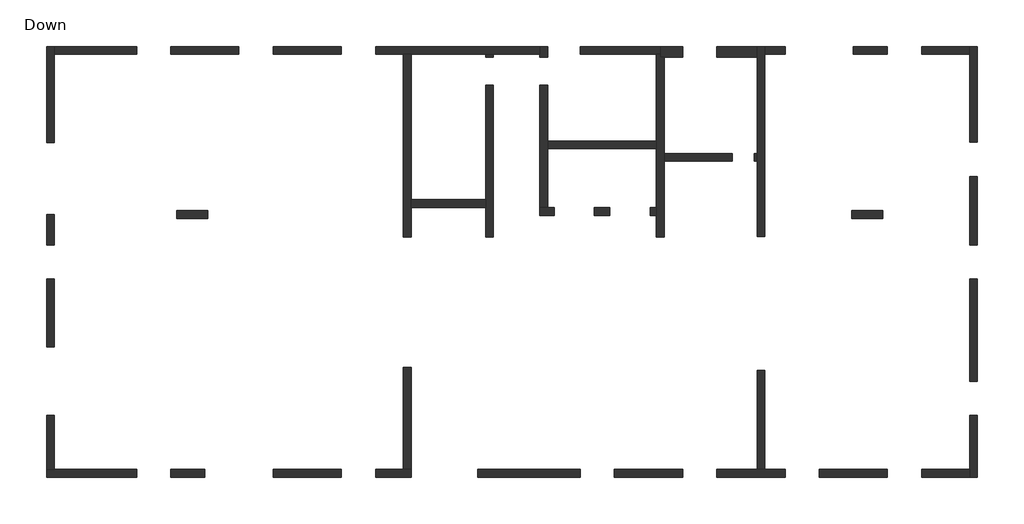
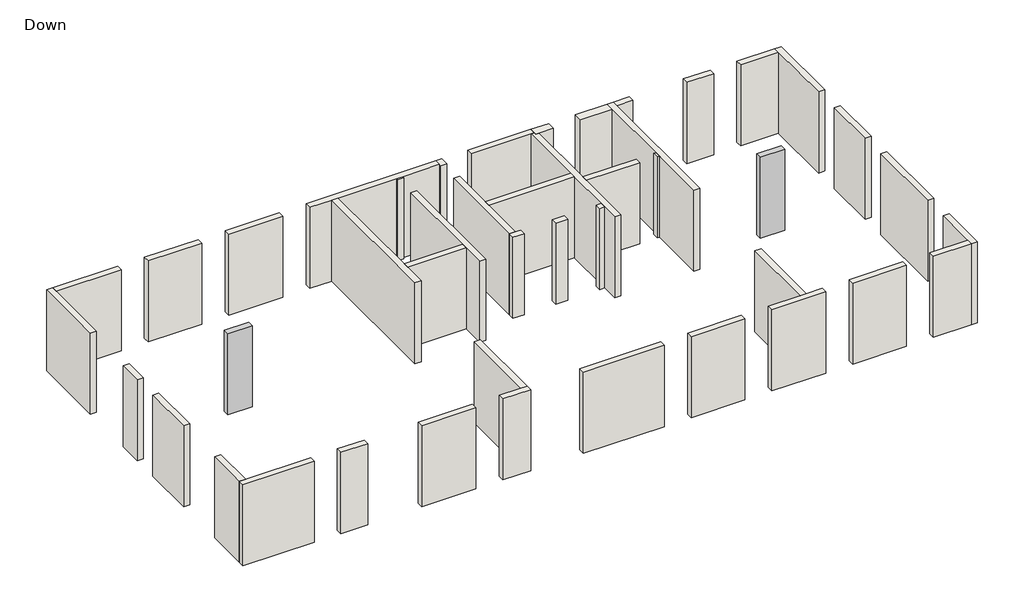
# One storey: 43 walls, 2 columns.
"""IFC4 building model written with IfcOpenShell, lengths in millimetres."""

from ifc_helpers import new_model, si_unit, origin, origin_with_axes, place, context, project, spatial, polyline, outline, extrude, faceted_brep, element, save

model = new_model("IFC4")

# Units and contexts
model_context = context("Model", 3, world=origin())
ifc_project = project(units=[si_unit("LENGTHUNIT", "METRE", prefix="MILLI")], contexts=[model_context])

# Site, building, storey
site = spatial("IfcSite", under=ifc_project)
building = spatial("IfcBuilding", under=site)
storey = spatial("IfcBuildingStorey", under=building, Name="Down", Elevation=0.0)

# Columns
placement = place(None, origin())
element("IfcColumn", 1, ObjectType="Concrete Rectengular Column : 100/25", at=placement, inside=storey, context=model_context, shape_type="Brep", body=[
    faceted_brep([(-7230.8224108, 3391.6516226, 0.0), (-6230.8224108, 3391.6516226, 0.0), (-6230.8224108, 3141.6516226, 0.0), (-7230.8224108, 3141.6516226, 0.0), (-7230.8224108, 3391.6516226, 3500.0), (-6230.8224108, 3391.6516226, 3500.0), (-6230.8224108, 3391.6516226, 3290.0), (-7230.8224108, 3391.6516226, 3290.0), (-6230.8224108, 3141.6516226, 3500.0), (-6230.8224108, 3141.6516226, 3290.0), (-7230.8224108, 3141.6516226, 3500.0), (-7230.8224108, 3141.6516226, 3290.0)], [[[0, 1, 2, 3]], [[4, 5, 6, 1, 0, 7]], [[5, 8, 9, 2, 1, 6]], [[8, 10, 11, 3, 2, 9]], [[10, 4, 7, 0, 3, 11]], [[4, 10, 8, 5]]]),
])
element("IfcColumn", 2, ObjectType="Concrete Rectengular Column : 100/25", at=placement, inside=storey, context=model_context, shape_type="Brep", body=[
    faceted_brep([(14515.7915847, 3391.6516226, 0.0), (15515.7915847, 3391.6516226, 0.0), (15515.7915847, 3141.6516226, 0.0), (14515.7915847, 3141.6516226, 0.0), (14515.7915847, 3391.6516226, 3500.0), (15515.7915847, 3391.6516226, 3500.0), (15515.7915847, 3391.6516226, 3290.0), (14515.7915847, 3391.6516226, 3290.0), (15515.7915847, 3141.6516226, 3500.0), (15515.7915847, 3141.6516226, 3290.0), (14515.7915847, 3141.6516226, 3500.0), (14515.7915847, 3141.6516226, 3290.0)], [[[0, 1, 2, 3]], [[4, 5, 6, 1, 0, 7]], [[5, 8, 9, 2, 1, 6]], [[8, 10, 11, 3, 2, 9]], [[10, 4, 7, 0, 3, 11]], [[4, 10, 8, 5]]]),
])

# Walls
element("IfcWall", 3, ObjectType="25", at=placement, inside=storey, context=model_context, shape_type="Brep", body=[
    faceted_brep([(18317.4281535, 8690.4665211, 0.0), (18317.4281535, 8440.4665211, 0.0), (18317.4281535, 5600.7374014, 0.0), (18317.4281535, 5600.7374014, 3500.0), (18317.4281535, 8440.4665211, 3500.0), (18317.4281535, 8690.4665211, 3500.0), (18567.4281535, 8690.4665211, 0.0), (18567.4281535, 8690.4665211, 3500.0), (18567.4281535, 5600.7374014, 3500.0), (18567.4281535, 5600.7374014, 0.0)], [[[0, 1, 2, 3, 4, 5]], [[6, 7, 8, 9]], [[2, 1, 0, 6, 9]], [[3, 2, 9, 8]], [[5, 4, 3, 8, 7]], [[0, 5, 7, 6]]]),
])
element("IfcWall", 4, ObjectType="25", at=placement, inside=storey, context=model_context, shape_type="SweptSolid", body=[
    extrude(outline(polyline([(18317.4281535, 2290.9179883), (18317.4281535, 4491.8209229), (18567.4281535, 4491.8209229), (18567.4281535, 2290.9179883), (18317.4281535, 2290.9179883)])), origin_with_axes(), (0.0, 0.0, 1.0), 3500.0),
])
element("IfcWall", 5, ObjectType="25", at=placement, inside=storey, context=model_context, shape_type="SweptSolid", body=[
    extrude(outline(polyline([(18317.4281535, -2106.6553751), (18317.4281535, 1194.6990267), (18567.4281535, 1194.6990267), (18567.4281535, -2106.6553751), (18317.4281535, -2106.6553751)])), origin_with_axes(), (0.0, 0.0, 1.0), 3500.0),
])
element("IfcWall", 6, ObjectType="25", at=placement, inside=storey, context=model_context, shape_type="Brep", body=[
    faceted_brep([(18317.4281535, -3207.1068424, 0.0), (18317.4281535, -4954.849506, 0.0), (18317.4281535, -5204.849506, 0.0), (18317.4281535, -5204.849506, 3500.0), (18317.4281535, -4954.849506, 3500.0), (18317.4281535, -3207.1068424, 3500.0), (18567.4281535, -3207.1068424, 0.0), (18567.4281535, -3207.1068424, 3500.0), (18567.4281535, -5204.849506, 3500.0), (18567.4281535, -5204.849506, 0.0)], [[[0, 1, 2, 3, 4, 5]], [[6, 7, 8, 9]], [[2, 1, 0, 6, 9]], [[5, 4, 3, 8, 7]], [[0, 5, 7, 6]], [[3, 2, 9, 8]]]),
])
element("IfcWall", 7, ObjectType="25", at=placement, inside=storey, context=model_context, shape_type="Brep", body=[
    faceted_brep([(18317.4281535, -4954.849506, 0.0), (16768.6132551, -4954.849506, 0.0), (16768.6132551, -4954.849506, 3500.0), (18317.4281535, -4954.849506, 3500.0), (18317.4281535, -4954.849506, 3290.0), (18317.4281535, -5204.849506, 0.0), (18317.4281535, -5204.849506, 3500.0), (16768.6132551, -5204.849506, 3500.0), (16768.6132551, -5204.849506, 0.0)], [[[0, 1, 2, 3, 4]], [[5, 6, 7, 8]], [[1, 0, 5, 8]], [[2, 1, 8, 7]], [[3, 2, 7, 6]], [[0, 4, 3, 6, 5]]]),
])
element("IfcWall", 8, ObjectType="25", at=placement, inside=storey, context=model_context, shape_type="SweptSolid", body=[
    extrude(outline(polyline([(13467.2588533, -4954.849506), (15668.1617879, -4954.849506), (15668.1617879, -5204.849506), (13467.2588533, -5204.849506), (13467.2588533, -4954.849506)])), origin_with_axes(), (0.0, 0.0, 1.0), 3500.0),
])
element("IfcWall", 9, ObjectType="25", at=placement, inside=storey, context=model_context, shape_type="Brep", body=[
    faceted_brep([(12366.8073861, -4954.849506, 0.0), (11719.2340226, -4954.849506, 0.0), (11469.2340226, -4954.849506, 0.0), (10165.9044515, -4954.849506, 0.0), (10165.9044515, -4954.849506, 3500.0), (11469.2340226, -4954.849506, 3500.0), (11719.2340226, -4954.849506, 3500.0), (12366.8073861, -4954.849506, 3500.0), (12366.8073861, -5204.849506, 0.0), (12366.8073861, -5204.849506, 3500.0), (10165.9044515, -5204.849506, 3500.0), (10165.9044515, -5204.849506, 0.0)], [[[0, 1, 2, 3, 4, 5, 6, 7]], [[8, 9, 10, 11]], [[3, 2, 1, 0, 8, 11]], [[4, 3, 11, 10]], [[7, 6, 5, 4, 10, 9]], [[0, 7, 9, 8]]]),
])
element("IfcWall", 10, ObjectType="25", at=placement, inside=storey, context=model_context, shape_type="SweptSolid", body=[
    extrude(outline(polyline([(6868.7825554, -4954.849506), (9069.6854899, -4954.849506), (9069.6854899, -5204.849506), (6868.7825554, -5204.849506), (6868.7825554, -4954.849506)])), origin_with_axes(), (0.0, 0.0, 1.0), 3500.0),
])
element("IfcWall", 11, ObjectType="25", at=placement, inside=storey, context=model_context, shape_type="SweptSolid", body=[
    extrude(outline(polyline([(2466.9766863, -4954.849506), (5768.3310881, -4954.849506), (5768.3310881, -5204.849506), (2466.9766863, -5204.849506), (2466.9766863, -4954.849506)])), origin_with_axes(), (0.0, 0.0, 1.0), 3500.0),
])
element("IfcWall", 12, ObjectType="25", at=placement, inside=storey, context=model_context, shape_type="Brep", body=[
    faceted_brep([(317.1459865, -4954.849506, 0.0), (67.1459865, -4954.849506, 0.0), (-830.1452099, -4954.849506, 0.0), (-830.1452099, -4954.849506, 3500.0), (67.1459865, -4954.849506, 3500.0), (317.1459865, -4954.849506, 3500.0), (317.1459865, -5204.849506, 0.0), (317.1459865, -5204.849506, 3500.0), (-830.1452099, -5204.849506, 3500.0), (-830.1452099, -5204.849506, 0.0)], [[[0, 1, 2, 3, 4, 5]], [[6, 7, 8, 9]], [[2, 1, 0, 6, 9]], [[3, 2, 9, 8]], [[5, 4, 3, 8, 7]], [[0, 5, 7, 6]]]),
])
element("IfcWall", 13, ObjectType="25", at=placement, inside=storey, context=model_context, shape_type="SweptSolid", body=[
    extrude(outline(polyline([(-4131.4996117, -4954.849506), (-1930.5966772, -4954.849506), (-1930.5966772, -5204.849506), (-4131.4996117, -5204.849506), (-4131.4996117, -4954.849506)])), origin_with_axes(), (0.0, 0.0, 1.0), 3500.0),
])
element("IfcWall", 14, ObjectType="25", at=placement, inside=storey, context=model_context, shape_type="SweptSolid", body=[
    extrude(outline(polyline([(-7432.8540135, -4954.849506), (-6332.4025462, -4954.849506), (-6332.4025462, -5204.849506), (-7432.8540135, -5204.849506), (-7432.8540135, -4954.849506)])), origin_with_axes(), (0.0, 0.0, 1.0), 3500.0),
])
element("IfcWall", 15, ObjectType="25", at=placement, inside=storey, context=model_context, shape_type="Brep", body=[
    faceted_brep([(-8529.0729751, -4954.849506, 0.0), (-11182.5718465, -4954.849506, 0.0), (-11432.5718465, -4954.849506, 0.0), (-11432.5718465, -4954.849506, 3500.0), (-11182.5718465, -4954.849506, 3500.0), (-8529.0729751, -4954.849506, 3500.0), (-8529.0729751, -5204.849506, 0.0), (-8529.0729751, -5204.849506, 3500.0), (-11432.5718465, -5204.849506, 3500.0), (-11432.5718465, -5204.849506, 0.0)], [[[0, 1, 2, 3, 4, 5]], [[6, 7, 8, 9]], [[2, 1, 0, 6, 9]], [[5, 4, 3, 8, 7]], [[0, 5, 7, 6]], [[3, 2, 9, 8]]]),
])
element("IfcWall", 16, ObjectType="25", at=placement, inside=storey, context=model_context, shape_type="Brep", body=[
    faceted_brep([(-11182.5718465, -4954.849506, 0.0), (-11182.5718465, -3207.1068424, 0.0), (-11182.5718465, -3207.1068424, 3290.0), (-11182.5718465, -3207.1068424, 3500.0), (-11182.5718465, -4954.849506, 3500.0), (-11182.5718465, -4954.849506, 3290.0), (-11432.5718465, -4954.849506, 0.0), (-11432.5718465, -4954.849506, 3500.0), (-11432.5718465, -3207.1068424, 3500.0), (-11432.5718465, -3207.1068424, 0.0), (-11187.5718465, -3207.1068424, 3500.0)], [[[0, 1, 2, 3, 4, 5]], [[6, 7, 8, 9]], [[1, 0, 6, 9]], [[3, 2, 1, 9, 8, 10]], [[4, 3, 10, 8, 7]], [[0, 5, 4, 7, 6]]]),
])
element("IfcWall", 17, ObjectType="25", at=placement, inside=storey, context=model_context, shape_type="Brep", body=[
    faceted_brep([(-11182.5718465, -1006.2039078, 0.0), (-11182.5718465, 1194.6990267, 0.0), (-11182.5718465, 1194.6990267, 3290.0), (-11182.5718465, 1194.6990267, 3500.0), (-11182.5718465, -1006.2039078, 3500.0), (-11182.5718465, -1006.2039078, 3290.0), (-11432.5718465, -1006.2039078, 0.0), (-11432.5718465, -1006.2039078, 3500.0), (-11432.5718465, 1194.6990267, 3500.0), (-11432.5718465, 1194.6990267, 0.0), (-11187.5718465, 1194.6990267, 3500.0), (-11187.5718465, -1006.2039078, 3500.0)], [[[0, 1, 2, 3, 4, 5]], [[6, 7, 8, 9]], [[1, 0, 6, 9]], [[3, 2, 1, 9, 8, 10]], [[4, 3, 10, 8, 7, 11]], [[0, 5, 4, 11, 7, 6]]]),
])
element("IfcWall", 18, ObjectType="25", at=placement, inside=storey, context=model_context, shape_type="Brep", body=[
    faceted_brep([(-11182.5718465, 2290.9179883, 0.0), (-11182.5718465, 3268.626792, 0.0), (-11182.5718465, 3268.626792, 3290.0), (-11182.5718465, 3268.626792, 3500.0), (-11182.5718465, 2290.9179883, 3500.0), (-11182.5718465, 2290.9179883, 3290.0), (-11432.5718465, 2290.9179883, 0.0), (-11432.5718465, 2290.9179883, 3500.0), (-11432.5718465, 3268.626792, 3500.0), (-11432.5718465, 3268.626792, 0.0), (-11187.5718465, 3268.626792, 3500.0), (-11187.5718465, 2290.9179883, 3500.0)], [[[0, 1, 2, 3, 4, 5]], [[6, 7, 8, 9]], [[1, 0, 6, 9]], [[3, 2, 1, 9, 8, 10]], [[4, 3, 10, 8, 7, 11]], [[0, 5, 4, 11, 7, 6]]]),
])
element("IfcWall", 19, ObjectType="25", at=placement, inside=storey, context=model_context, shape_type="Brep", body=[
    faceted_brep([(-11182.5718465, 5592.2723901, 0.0), (-11182.5718465, 8440.4665211, 0.0), (-11182.5718465, 8690.4665211, 0.0), (-11182.5718465, 8690.4665211, 3500.0), (-11182.5718465, 8440.4665211, 3500.0), (-11182.5718465, 5592.2723901, 3500.0), (-11182.5718465, 5592.2723901, 3290.0), (-11432.5718465, 5592.2723901, 0.0), (-11432.5718465, 5592.2723901, 3500.0), (-11432.5718465, 8690.4665211, 3500.0), (-11432.5718465, 8690.4665211, 0.0), (-11187.5718465, 5592.2723901, 3500.0)], [[[0, 1, 2, 3, 4, 5, 6]], [[7, 8, 9, 10]], [[2, 1, 0, 7, 10]], [[5, 4, 3, 9, 8, 11]], [[0, 6, 5, 11, 8, 7]], [[3, 2, 10, 9]]]),
])
element("IfcWall", 20, ObjectType="25", at=placement, inside=storey, context=model_context, shape_type="Brep", body=[
    faceted_brep([(-11182.5718465, 8440.4665211, 0.0), (-8529.0729751, 8440.4665211, 0.0), (-8529.0729751, 8440.4665211, 3500.0), (-11182.5718465, 8440.4665211, 3500.0), (-11182.5718465, 8440.4665211, 3290.0), (-11182.5718465, 8690.4665211, 0.0), (-11182.5718465, 8690.4665211, 3500.0), (-8529.0729751, 8690.4665211, 3500.0), (-8529.0729751, 8690.4665211, 0.0)], [[[0, 1, 2, 3, 4]], [[5, 6, 7, 8]], [[1, 0, 5, 8]], [[2, 1, 8, 7]], [[3, 2, 7, 6]], [[0, 4, 3, 6, 5]]]),
])
element("IfcWall", 21, ObjectType="25", at=placement, inside=storey, context=model_context, shape_type="SweptSolid", body=[
    extrude(outline(polyline([(-5232.8540135, 8440.4665211), (-7432.8540135, 8440.4665211), (-7432.8540135, 8690.4665211), (-5232.8540135, 8690.4665211), (-5232.8540135, 8440.4665211)])), origin_with_axes(), (0.0, 0.0, 1.0), 3500.0),
])
element("IfcWall", 22, ObjectType="25", at=placement, inside=storey, context=model_context, shape_type="SweptSolid", body=[
    extrude(outline(polyline([(-1930.5966772, 8440.4665211), (-4131.4996117, 8440.4665211), (-4131.4996117, 8690.4665211), (-1930.5966772, 8690.4665211), (-1930.5966772, 8440.4665211)])), origin_with_axes(), (0.0, 0.0, 1.0), 3500.0),
])
element("IfcWall", 23, ObjectType="25", at=placement, inside=storey, context=model_context, shape_type="Brep", body=[
    faceted_brep([(-830.1452099, 8440.4665211, 0.0), (67.1459865, 8440.4665211, 0.0), (317.1459865, 8440.4665211, 0.0), (2716.4123522, 8440.4665211, 0.0), (2966.4123522, 8440.4665211, 0.0), (4468.6696885, 8440.4665211, 0.0), (4468.6696885, 8440.4665211, 3290.0), (4468.6696885, 8440.4665211, 3500.0), (2966.4123522, 8440.4665211, 3500.0), (2716.4123522, 8440.4665211, 3500.0), (317.1459865, 8440.4665211, 3500.0), (67.1459865, 8440.4665211, 3500.0), (-830.1452099, 8440.4665211, 3500.0), (-830.1452099, 8690.4665211, 0.0), (-830.1452099, 8690.4665211, 3500.0), (4468.6696885, 8690.4665211, 3500.0), (4468.6696885, 8690.4665211, 0.0)], [[[0, 1, 2, 3, 4, 5, 6, 7, 8, 9, 10, 11, 12]], [[13, 14, 15, 16]], [[5, 4, 3, 2, 1, 0, 13, 16]], [[12, 11, 10, 9, 8, 7, 15, 14]], [[0, 12, 14, 13]], [[7, 6, 5, 16, 15]]]),
])
element("IfcWall", 24, ObjectType="25", at=placement, inside=storey, context=model_context, shape_type="Brep", body=[
    faceted_brep([(4468.6696885, 8690.4665211, 0.0), (4468.6696885, 8440.4665211, 0.0), (4468.6696885, 8343.4010583, 0.0), (4468.6696885, 8343.4010583, 3290.0), (4468.6696885, 8343.4010583, 3500.0), (4468.6696885, 8440.4665211, 3500.0), (4468.6696885, 8690.4665211, 3500.0), (4718.6696885, 8690.4665211, 0.0), (4718.6696885, 8690.4665211, 3500.0), (4718.6696885, 8445.4665211, 3500.0), (4718.6696885, 8343.4010583, 3500.0), (4718.6696885, 8343.4010583, 3290.0), (4718.6696885, 8343.4010583, 0.0)], [[[0, 1, 2, 3, 4, 5, 6]], [[7, 8, 9, 10, 11, 12]], [[2, 1, 0, 7, 12]], [[4, 3, 2, 12, 11, 10]], [[6, 5, 4, 10, 9, 8]], [[0, 6, 8, 7]]]),
])
element("IfcWall", 25, ObjectType="25", at=placement, inside=storey, context=model_context, shape_type="Brep", body=[
    faceted_brep([(2966.4123522, 8343.4010583, 0.0), (2966.4123522, 8440.4665211, 0.0), (2966.4123522, 8440.4665211, 3290.0), (2966.4123522, 8440.4665211, 3500.0), (2966.4123522, 8343.4010583, 3500.0), (2966.4123522, 8343.4010583, 3290.0), (2716.4123522, 8343.4010583, 0.0), (2716.4123522, 8343.4010583, 3290.0), (2716.4123522, 8343.4010583, 3500.0), (2716.4123522, 8440.4665211, 3500.0), (2716.4123522, 8440.4665211, 0.0)], [[[0, 1, 2, 3, 4, 5]], [[6, 7, 8, 9, 10]], [[1, 0, 6, 10]], [[4, 3, 9, 8]], [[0, 5, 4, 8, 7, 6]], [[3, 2, 1, 10, 9]]]),
])
element("IfcWall", 26, ObjectType="25", at=placement, inside=storey, context=model_context, shape_type="Brep", body=[
    faceted_brep([(67.1459865, 8440.4665211, 0.0), (67.1459865, 2544.8683269, 0.0), (67.1459865, 2544.8683269, 3290.0), (67.1459865, 2544.8683269, 3500.0), (67.1459865, 8440.4665211, 3500.0), (67.1459865, 8440.4665211, 3290.0), (317.1459865, 8440.4665211, 0.0), (317.1459865, 8440.4665211, 3500.0), (317.1459865, 3751.1324353, 3500.0), (317.1459865, 3501.1324353, 3500.0), (317.1459865, 2544.8683269, 3500.0), (317.1459865, 2544.8683269, 0.0), (317.1459865, 3501.1324353, 0.0), (317.1459865, 3751.1324353, 0.0)], [[[0, 1, 2, 3, 4, 5]], [[6, 7, 8, 9, 10, 11, 12, 13]], [[1, 0, 6, 13, 12, 11]], [[3, 2, 1, 11, 10]], [[4, 3, 10, 9, 8, 7]], [[0, 5, 4, 7, 6]]]),
])
element("IfcWall", 27, ObjectType="25", at=placement, inside=storey, context=model_context, shape_type="Brep", body=[
    faceted_brep([(2966.4123522, 2544.8683269, 0.0), (2966.4123522, 7441.8773563, 0.0), (2966.4123522, 7441.8773563, 3290.0), (2966.4123522, 7441.8773563, 3500.0), (2966.4123522, 2544.8683269, 3500.0), (2966.4123522, 2544.8683269, 3290.0), (2716.4123522, 2544.8683269, 0.0), (2716.4123522, 2544.8683269, 3500.0), (2716.4123522, 3501.1324353, 3500.0), (2716.4123522, 3751.1324353, 3500.0), (2716.4123522, 7441.8773563, 3500.0), (2716.4123522, 7441.8773563, 3290.0), (2716.4123522, 7441.8773563, 0.0), (2716.4123522, 3751.1324353, 0.0), (2716.4123522, 3501.1324353, 0.0)], [[[0, 1, 2, 3, 4, 5]], [[6, 7, 8, 9, 10, 11, 12, 13, 14]], [[1, 0, 6, 14, 13, 12]], [[3, 2, 1, 12, 11, 10]], [[4, 3, 10, 9, 8, 7]], [[0, 5, 4, 7, 6]]]),
])
element("IfcWall", 28, ObjectType="25", at=placement, inside=storey, context=model_context, shape_type="SweptSolid", body=[
    extrude(outline(polyline([(2716.4123522, 3501.1324353), (317.1459865, 3501.1324353), (317.1459865, 3751.1324353), (2716.4123522, 3751.1324353), (2716.4123522, 3501.1324353)])), origin_with_axes(), (0.0, 0.0, 1.0), 3500.0),
])
element("IfcWall", 29, ObjectType="25", at=placement, inside=storey, context=model_context, shape_type="Brep", body=[
    faceted_brep([(4718.9518556, 3493.2317581, 0.0), (4718.9518556, 5393.0624579, 0.0), (4718.9518556, 5643.0624579, 0.0), (4718.9518556, 7441.8773563, 0.0), (4718.9518556, 7441.8773563, 3290.0), (4718.9518556, 7441.8773563, 3500.0), (4718.9518556, 5643.0624579, 3500.0), (4718.9518556, 5393.0624579, 3500.0), (4718.9518556, 3493.2317581, 3500.0), (4468.9518556, 3493.2317581, 0.0), (4468.9518556, 3493.2317581, 3500.0), (4468.9518556, 7441.8773563, 3500.0), (4468.9518556, 7441.8773563, 3290.0), (4468.9518556, 7441.8773563, 0.0), (4718.6696885, 7441.8773563, 3500.0)], [[[0, 1, 2, 3, 4, 5, 6, 7, 8]], [[9, 10, 11, 12, 13]], [[3, 2, 1, 0, 9, 13]], [[5, 4, 3, 13, 12, 11, 14]], [[8, 7, 6, 5, 14, 11, 10]], [[0, 8, 10, 9]]]),
])
element("IfcWall", 30, ObjectType="25", at=placement, inside=storey, context=model_context, shape_type="Brep", body=[
    faceted_brep([(4468.9518556, 3243.2317581, 0.0), (4926.0624651, 3243.2317581, 0.0), (4926.0624651, 3243.2317581, 3290.0), (4926.0624651, 3243.2317581, 3500.0), (4468.9518556, 3243.2317581, 3500.0), (4468.9518556, 3243.2317581, 3290.0), (4468.9518556, 3493.2317581, 0.0), (4468.9518556, 3493.2317581, 3500.0), (4718.9518556, 3493.2317581, 3500.0), (4926.0624651, 3493.2317581, 3500.0), (4926.0624651, 3493.2317581, 3290.0), (4926.0624651, 3493.2317581, 0.0), (4718.9518556, 3493.2317581, 0.0)], [[[0, 1, 2, 3, 4, 5]], [[6, 7, 8, 9, 10, 11, 12]], [[1, 0, 6, 12, 11]], [[3, 2, 1, 11, 10, 9]], [[4, 3, 9, 8, 7]], [[0, 5, 4, 7, 6]]]),
])
element("IfcWall", 31, ObjectType="25", at=placement, inside=storey, context=model_context, shape_type="Brep", body=[
    faceted_brep([(6216.9766863, 3243.2317581, 0.0), (6716.4123522, 3243.2317581, 0.0), (6716.4123522, 3243.2317581, 3290.0), (6716.4123522, 3243.2317581, 3500.0), (6216.9766863, 3243.2317581, 3500.0), (6216.9766863, 3243.2317581, 3290.0), (6216.9766863, 3493.2317581, 0.0), (6216.9766863, 3493.2317581, 3290.0), (6216.9766863, 3493.2317581, 3500.0), (6716.4123522, 3493.2317581, 3500.0), (6716.4123522, 3493.2317581, 3290.0), (6716.4123522, 3493.2317581, 0.0)], [[[0, 1, 2, 3, 4, 5]], [[6, 7, 8, 9, 10, 11]], [[1, 0, 6, 11]], [[3, 2, 1, 11, 10, 9]], [[4, 3, 9, 8]], [[0, 5, 4, 8, 7, 6]]]),
])
element("IfcWall", 32, ObjectType="25", at=placement, inside=storey, context=model_context, shape_type="Brep", body=[
    faceted_brep([(8468.6696885, 2544.8683269, 0.0), (8468.6696885, 4990.9744217, 0.0), (8468.6696885, 5240.9744217, 0.0), (8468.6696885, 8340.4665211, 0.0), (8468.6696885, 8340.4665211, 3290.0), (8468.6696885, 8340.4665211, 3500.0), (8468.6696885, 5240.9744217, 3500.0), (8468.6696885, 4990.9744217, 3500.0), (8468.6696885, 2544.8683269, 3500.0), (8468.6696885, 2544.8683269, 3290.0), (8218.6696885, 2544.8683269, 0.0), (8218.6696885, 2544.8683269, 3290.0), (8218.6696885, 2544.8683269, 3500.0), (8218.6696885, 3243.2317581, 3500.0), (8218.6696885, 3493.2317581, 3500.0), (8218.6696885, 5393.0624579, 3500.0), (8218.6696885, 5643.0624579, 3500.0), (8218.6696885, 8440.4665211, 3500.0), (8218.6696885, 8440.4665211, 3290.0), (8218.6696885, 8440.4665211, 0.0), (8218.6696885, 5643.0624579, 0.0), (8218.6696885, 5393.0624579, 0.0), (8218.6696885, 3493.2317581, 0.0), (8218.6696885, 3243.2317581, 0.0), (8343.6696885, 8440.4665211, 0.0), (8343.6696885, 8340.4665211, 0.0), (8343.6696885, 8340.4665211, 3500.0), (8343.6696885, 8440.4665211, 3500.0)], [[[0, 1, 2, 3, 4, 5, 6, 7, 8, 9]], [[10, 11, 12, 13, 14, 15, 16, 17, 18, 19, 20, 21, 22, 23]], [[3, 2, 1, 0, 10, 23, 22, 21, 20, 19, 24, 25]], [[8, 7, 6, 5, 26, 27, 17, 16, 15, 14, 13, 12]], [[0, 9, 8, 12, 11, 10]], [[5, 4, 3, 25, 26]], [[25, 24, 27, 26]], [[24, 19, 18, 17, 27]]]),
])
element("IfcWall", 33, ObjectType="25", at=placement, inside=storey, context=model_context, shape_type="Brep", body=[
    faceted_brep([(8020.0240903, 3243.2317581, 0.0), (8218.6696885, 3243.2317581, 0.0), (8218.6696885, 3243.2317581, 3290.0), (8218.6696885, 3243.2317581, 3500.0), (8020.0240903, 3243.2317581, 3500.0), (8020.0240903, 3243.2317581, 3290.0), (8020.0240903, 3493.2317581, 0.0), (8020.0240903, 3493.2317581, 3290.0), (8020.0240903, 3493.2317581, 3500.0), (8218.6696885, 3493.2317581, 3500.0), (8218.6696885, 3493.2317581, 0.0)], [[[0, 1, 2, 3, 4, 5]], [[6, 7, 8, 9, 10]], [[1, 0, 6, 10]], [[4, 3, 9, 8]], [[0, 5, 4, 8, 7, 6]], [[3, 2, 1, 10, 9]]]),
])
element("IfcWall", 34, ObjectType="25", at=placement, inside=storey, context=model_context, shape_type="Brep", body=[
    faceted_brep([(4718.9518556, 5393.0624579, 0.0), (8218.6696885, 5393.0624579, 0.0), (8218.6696885, 5393.0624579, 3500.0), (4718.9518556, 5393.0624579, 3500.0), (4718.9518556, 5643.0624579, 0.0), (4718.9518556, 5643.0624579, 3290.0), (4718.9518556, 5643.0624579, 3500.0), (8218.6696885, 5643.0624579, 3500.0), (8218.6696885, 5643.0624579, 3290.0), (8218.6696885, 5643.0624579, 0.0)], [[[0, 1, 2, 3]], [[4, 5, 6, 7, 8, 9]], [[1, 0, 4, 9]], [[3, 2, 7, 6]], [[0, 3, 6, 5, 4]], [[2, 1, 9, 8, 7]]]),
])
element("IfcWall", 35, ObjectType="25", at=placement, inside=storey, context=model_context, shape_type="Brep", body=[
    faceted_brep([(5768.3310881, 8440.4665211, 0.0), (8218.6696885, 8440.4665211, 0.0), (8343.6696885, 8440.4665211, 0.0), (8343.6696885, 8440.4665211, 3500.0), (8218.6696885, 8440.4665211, 3500.0), (5768.3310881, 8440.4665211, 3500.0), (5768.3310881, 8440.4665211, 3290.0), (5768.3310881, 8690.4665211, 0.0), (5768.3310881, 8690.4665211, 3500.0), (8343.6696885, 8690.4665211, 3500.0), (8343.6696885, 8690.4665211, 0.0), (5768.3310881, 8445.4665211, 3500.0)], [[[0, 1, 2, 3, 4, 5, 6]], [[7, 8, 9, 10]], [[2, 1, 0, 7, 10]], [[3, 2, 10, 9]], [[5, 4, 3, 9, 8, 11]], [[0, 6, 5, 11, 8, 7]]]),
])
element("IfcWall", 36, ObjectType="25", at=placement, inside=storey, context=model_context, shape_type="Brep", body=[
    faceted_brep([(8468.6696885, 4990.9744217, 0.0), (10669.5726231, 4990.9744217, 0.0), (10669.5726231, 4990.9744217, 3290.0), (10669.5726231, 4990.9744217, 3500.0), (8468.6696885, 4990.9744217, 3500.0), (8468.6696885, 4990.9744217, 3290.0), (8468.6696885, 5240.9744217, 0.0), (8468.6696885, 5240.9744217, 3290.0), (8468.6696885, 5240.9744217, 3500.0), (10669.5726231, 5240.9744217, 3500.0), (10669.5726231, 5240.9744217, 3290.0), (10669.5726231, 5240.9744217, 0.0)], [[[0, 1, 2, 3, 4, 5]], [[6, 7, 8, 9, 10, 11]], [[1, 0, 6, 11]], [[3, 2, 1, 11, 10, 9]], [[4, 3, 9, 8]], [[0, 5, 4, 8, 7, 6]]]),
])
element("IfcWall", 37, ObjectType="25", at=placement, inside=storey, context=model_context, shape_type="Brep", body=[
    faceted_brep([(11719.2340226, 2566.0308552, 0.0), (11719.2340226, 8440.7486881, 0.0), (11719.2340226, 8690.7486881, 0.0), (11719.2340226, 8690.7486881, 3500.0), (11719.2340226, 8440.7486881, 3500.0), (11719.2340226, 2566.0308552, 3500.0), (11719.2340226, 2566.0308552, 3290.0), (11469.2340226, 2566.0308552, 0.0), (11469.2340226, 2566.0308552, 3290.0), (11469.2340226, 2566.0308552, 3500.0), (11469.2340226, 4991.2565888, 3500.0), (11469.2340226, 5241.2565888, 3500.0), (11469.2340226, 8340.4665211, 3500.0), (11469.2340226, 8690.4665211, 3500.0), (11469.2340226, 8690.7486881, 3500.0), (11469.2340226, 8690.7486881, 0.0), (11469.2340226, 8690.4665211, 0.0), (11469.2340226, 8340.4665211, 0.0), (11469.2340226, 5241.2565888, 0.0), (11469.2340226, 4991.2565888, 0.0)], [[[0, 1, 2, 3, 4, 5, 6]], [[7, 8, 9, 10, 11, 12, 13, 14, 15, 16, 17, 18, 19]], [[2, 1, 0, 7, 19, 18, 17, 16, 15]], [[5, 4, 3, 14, 13, 12, 11, 10, 9]], [[0, 6, 5, 9, 8, 7]], [[3, 2, 15, 14]]]),
])
element("IfcWall", 38, ObjectType="25", at=placement, inside=storey, context=model_context, shape_type="Brep", body=[
    faceted_brep([(11719.2340226, 8440.7486881, 0.0), (12366.8073861, 8440.7486881, 0.0), (12366.8073861, 8440.7486881, 3500.0), (11719.2340226, 8440.7486881, 3500.0), (11719.2340226, 8440.7486881, 3290.0), (11719.2340226, 8690.7486881, 0.0), (11719.2340226, 8690.7486881, 3500.0), (12366.8073861, 8690.7486881, 3500.0), (12366.8073861, 8690.7486881, 0.0)], [[[0, 1, 2, 3, 4]], [[5, 6, 7, 8]], [[1, 0, 5, 8]], [[2, 1, 8, 7]], [[3, 2, 7, 6]], [[0, 4, 3, 6, 5]]]),
])
element("IfcWall", 39, ObjectType="25", at=placement, inside=storey, context=model_context, shape_type="Brep", body=[
    faceted_brep([(11372.1685599, 4991.2565888, 0.0), (11469.2340226, 4991.2565888, 0.0), (11469.2340226, 4991.2565888, 3290.0), (11469.2340226, 4991.2565888, 3500.0), (11372.1685599, 4991.2565888, 3500.0), (11372.1685599, 4991.2565888, 3290.0), (11372.1685599, 5241.2565888, 0.0), (11372.1685599, 5241.2565888, 3290.0), (11372.1685599, 5241.2565888, 3500.0), (11469.2340226, 5241.2565888, 3500.0), (11469.2340226, 5241.2565888, 3290.0), (11469.2340226, 5241.2565888, 0.0), (11372.1685599, 5240.9744217, 3500.0)], [[[0, 1, 2, 3, 4, 5]], [[6, 7, 8, 9, 10, 11]], [[1, 0, 6, 11]], [[4, 3, 9, 8, 12]], [[0, 5, 4, 12, 8, 7, 6]], [[3, 2, 1, 11, 10, 9]]]),
])
element("IfcWall", 40, ObjectType="25", at=placement, inside=storey, context=model_context, shape_type="Brep", body=[
    faceted_brep([(14567.7103206, 8440.4665211, 0.0), (15668.1617879, 8440.4665211, 0.0), (15668.1617879, 8440.4665211, 3290.0), (15668.1617879, 8440.4665211, 3500.0), (14567.7103206, 8440.4665211, 3500.0), (14567.7103206, 8440.4665211, 3290.0), (14567.7103206, 8690.4665211, 0.0), (14567.7103206, 8690.4665211, 3500.0), (15668.1617879, 8690.4665211, 3500.0), (15668.1617879, 8690.4665211, 0.0), (15668.1617879, 8440.7486881, 3500.0), (14567.7103206, 8440.7486881, 3500.0)], [[[0, 1, 2, 3, 4, 5]], [[6, 7, 8, 9]], [[1, 0, 6, 9]], [[3, 2, 1, 9, 8, 10]], [[4, 3, 10, 8, 7, 11]], [[0, 5, 4, 11, 7, 6]]]),
])
element("IfcWall", 41, ObjectType="25", at=placement, inside=storey, context=model_context, shape_type="Brep", body=[
    faceted_brep([(16768.6132551, 8440.4665211, 0.0), (18317.4281535, 8440.4665211, 0.0), (18317.4281535, 8440.4665211, 3290.0), (18317.4281535, 8440.4665211, 3500.0), (16768.6132551, 8440.4665211, 3500.0), (16768.6132551, 8440.4665211, 3290.0), (16768.6132551, 8690.4665211, 0.0), (16768.6132551, 8690.4665211, 3500.0), (18317.4281535, 8690.4665211, 3500.0), (18317.4281535, 8690.4665211, 0.0), (16768.6132551, 8440.7486881, 3500.0)], [[[0, 1, 2, 3, 4, 5]], [[6, 7, 8, 9]], [[1, 0, 6, 9]], [[4, 3, 8, 7, 10]], [[0, 5, 4, 10, 7, 6]], [[3, 2, 1, 9, 8]]]),
])
element("IfcWall", 42, ObjectType="25", at=placement, inside=storey, context=model_context, shape_type="Brep", body=[
    faceted_brep([(317.1459865, -4954.849506, 0.0), (317.1459865, -1658.0097769, 0.0), (317.1459865, -1658.0097769, 3290.0), (317.1459865, -1658.0097769, 3500.0), (317.1459865, -4954.849506, 3500.0), (317.1459865, -4954.849506, 3290.0), (67.1459865, -4954.849506, 0.0), (67.1459865, -4954.849506, 3290.0), (67.1459865, -4954.849506, 3500.0), (67.1459865, -1658.0097769, 3500.0), (67.1459865, -1658.0097769, 3290.0), (67.1459865, -1658.0097769, 0.0)], [[[0, 1, 2, 3, 4, 5]], [[6, 7, 8, 9, 10, 11]], [[1, 0, 6, 11]], [[3, 2, 1, 11, 10, 9]], [[4, 3, 9, 8]], [[0, 5, 4, 8, 7, 6]]]),
])
element("IfcWall", 43, ObjectType="25", at=placement, inside=storey, context=model_context, shape_type="Brep", body=[
    faceted_brep([(11719.2340226, -4954.849506, 0.0), (11719.2340226, -1755.3574067, 0.0), (11719.2340226, -1755.3574067, 3290.0), (11719.2340226, -1755.3574067, 3500.0), (11719.2340226, -4954.849506, 3500.0), (11719.2340226, -4954.849506, 3290.0), (11469.2340226, -4954.849506, 0.0), (11469.2340226, -4954.849506, 3290.0), (11469.2340226, -4954.849506, 3500.0), (11469.2340226, -1755.3574067, 3500.0), (11469.2340226, -1755.3574067, 3290.0), (11469.2340226, -1755.3574067, 0.0)], [[[0, 1, 2, 3, 4, 5]], [[6, 7, 8, 9, 10, 11]], [[1, 0, 6, 11]], [[3, 2, 1, 11, 10, 9]], [[4, 3, 9, 8]], [[0, 5, 4, 8, 7, 6]]]),
])
element("IfcWall", 44, ObjectType="35", at=placement, inside=storey, context=model_context, shape_type="Brep", body=[
    faceted_brep([(8343.6696885, 8340.4665211, 0.0), (8468.6696885, 8340.4665211, 0.0), (9069.6854899, 8340.4665211, 0.0), (9069.6854899, 8340.4665211, 3290.0), (9069.6854899, 8340.4665211, 3500.0), (8468.6696885, 8340.4665211, 3500.0), (8343.6696885, 8340.4665211, 3500.0), (8343.6696885, 8690.4665211, 0.0), (8343.6696885, 8690.4665211, 3500.0), (9069.6854899, 8690.4665211, 3500.0), (9069.6854899, 8690.4665211, 0.0), (8343.6696885, 8440.4665211, 0.0), (9069.6854899, 8345.4665211, 3500.0), (8343.6696885, 8440.4665211, 3500.0)], [[[0, 1, 2, 3, 4, 5, 6]], [[7, 8, 9, 10]], [[2, 1, 0, 11, 7, 10]], [[4, 3, 2, 10, 9, 12]], [[6, 5, 4, 12, 9, 8, 13]], [[0, 6, 13, 8, 7, 11]]]),
])
element("IfcWall", 45, ObjectType="35", at=placement, inside=storey, context=model_context, shape_type="Brep", body=[
    faceted_brep([(10165.9044515, 8340.4665211, 0.0), (11469.2340226, 8340.4665211, 0.0), (11469.2340226, 8340.4665211, 3290.0), (11469.2340226, 8340.4665211, 3500.0), (10165.9044515, 8340.4665211, 3500.0), (10165.9044515, 8340.4665211, 3290.0), (10165.9044515, 8690.4665211, 0.0), (10165.9044515, 8690.4665211, 3500.0), (11469.2340226, 8690.4665211, 3500.0), (11469.2340226, 8690.4665211, 0.0), (10165.9044515, 8345.4665211, 3500.0)], [[[0, 1, 2, 3, 4, 5]], [[6, 7, 8, 9]], [[1, 0, 6, 9]], [[4, 3, 8, 7, 10]], [[0, 5, 4, 10, 7, 6]], [[3, 2, 1, 9, 8]]]),
])

save(model, "model.ifc")

# Revit data of these elements
# Project information
#   Project Issue Date = "Issue Date"
#   Project Status = "Project Status"
#   Client Name = "לקוח"
#   Project Address = "Enter address here"
#   Project Name = "Project 005"
#   Project Number = "מספר פרויקט"
# Grids (mm)
#   "A": line (-11432.572, 10493.514) -> (-11432.572, -8726.294)
#   "B": line (-6730.258, 10493.514) -> (-6730.258, -8726.294)
#   "C": line (194.121, 10493.514) -> (194.121, -8726.294)
#   "D": line (2843.67, 10493.514) -> (2843.67, -8726.294)
#   "E": line (4591.695, 10493.514) -> (4591.695, -8726.294)
#   "F": line (8341.695, 10493.514) -> (8341.695, -8726.294)
#   "G": line (11592.259, 10493.514) -> (11592.259, -8726.294)
#   "H": line (18567.428, 10493.514) -> (18567.428, -8726.294)
#   "3": line (-14450.348, -5204.85) -> (22110.035, -5204.85)
#   "2": line (-14450.348, 3268.627) -> (22110.035, 3268.627)
#   "1": line (-14450.348, 8690.467) -> (22110.035, 8690.467)
# Type "Concrete Rectengular Column : 100/25"
#   b = 25 cm
#   h = 100 cm
#   Structural Material [instance default] = Concrete
# Type "25"
#   Layers, outside or top first: 25 cm "Concrete" (function 1)
# Type "35"
#   Layers, outside or top first: 35 cm "Concrete" (function 1)
# Element 1 (IfcColumn, "Concrete Rectengular Column : 100/25")
#   Comments = ""
#   Mark = "C1"
#   SOFiSTiK_AMG_Comments = ""
#   SOFiSTiK_AMG_Scheduled = yes
#   SOFiSTiK_AMG_Adjusted = yes
#   Structural Material = Concrete
#   Phase Created = New Construction
#   Materials on its faces: "Concrete"
# Element 2 (IfcColumn, "Concrete Rectengular Column : 100/25")
#   Comments = ""
#   Mark = "C2"
#   SOFiSTiK_AMG_Comments = ""
#   SOFiSTiK_AMG_Scheduled = yes
#   SOFiSTiK_AMG_Adjusted = yes
#   Structural Material = Concrete
#   Phase Created = New Construction
#   Materials on its faces: "Concrete"
# Element 3 (IfcWall, "25")
#   Comments = ""
#   Mark = "W1"
#   SOFiSTiK_AMG_Comments = ""
#   Top Offset = 0 cm
#   Base Offset = 0 cm
#   wall height = 350 cm
#   SOFiSTiK_AMG_Scheduled = yes
#   SOFiSTiK_AMG_Adjusted = yes
#   Phase Created = New Construction
#   Base Constraint = Down
#   Top Constraint = Typical Floor
#   Materials on its faces: "Concrete"
# Element 4 (IfcWall, "25")
#   Comments = ""
#   Mark = "W2"
#   SOFiSTiK_AMG_Comments = ""
#   Top Offset = 0 cm
#   Base Offset = 0 cm
#   wall height = 350 cm
#   SOFiSTiK_AMG_Scheduled = yes
#   SOFiSTiK_AMG_Adjusted = yes
#   Phase Created = New Construction
#   Base Constraint = Down
#   Top Constraint = Typical Floor
#   Materials on its faces: "Concrete"
# Element 5 (IfcWall, "25")
#   Comments = ""
#   Mark = "W3"
#   SOFiSTiK_AMG_Comments = ""
#   Top Offset = 0 cm
#   Base Offset = 0 cm
#   wall height = 350 cm
#   SOFiSTiK_AMG_Scheduled = yes
#   SOFiSTiK_AMG_Adjusted = yes
#   Phase Created = New Construction
#   Base Constraint = Down
#   Top Constraint = Typical Floor
#   Materials on its faces: "Concrete"
# Element 6 (IfcWall, "25")
#   Comments = ""
#   Mark = "W4"
#   SOFiSTiK_AMG_Comments = ""
#   Top Offset = 0 cm
#   Base Offset = 0 cm
#   wall height = 350 cm
#   SOFiSTiK_AMG_Scheduled = yes
#   SOFiSTiK_AMG_Adjusted = yes
#   Phase Created = New Construction
#   Base Constraint = Down
#   Top Constraint = Typical Floor
#   Materials on its faces: "Concrete"
# Element 7 (IfcWall, "25")
#   Comments = ""
#   Mark = "W5"
#   SOFiSTiK_AMG_Comments = ""
#   Top Offset = 0 cm
#   Base Offset = 0 cm
#   wall height = 350 cm
#   SOFiSTiK_AMG_Scheduled = yes
#   SOFiSTiK_AMG_Adjusted = yes
#   Phase Created = New Construction
#   Base Constraint = Down
#   Top Constraint = Typical Floor
#   Materials on its faces: "Concrete"
# Element 8 (IfcWall, "25")
#   Comments = ""
#   Mark = "W6"
#   SOFiSTiK_AMG_Comments = ""
#   Top Offset = 0 cm
#   Base Offset = 0 cm
#   wall height = 350 cm
#   SOFiSTiK_AMG_Scheduled = yes
#   SOFiSTiK_AMG_Adjusted = yes
#   Phase Created = New Construction
#   Base Constraint = Down
#   Top Constraint = Typical Floor
#   Materials on its faces: "Concrete"
# Element 9 (IfcWall, "25")
#   Comments = ""
#   Mark = "W7"
#   SOFiSTiK_AMG_Comments = ""
#   Top Offset = 0 cm
#   Base Offset = 0 cm
#   wall height = 350 cm
#   SOFiSTiK_AMG_Scheduled = yes
#   SOFiSTiK_AMG_Adjusted = yes
#   Phase Created = New Construction
#   Base Constraint = Down
#   Top Constraint = Typical Floor
#   Materials on its faces: "Concrete"
# Element 10 (IfcWall, "25")
#   Comments = ""
#   Mark = "W8"
#   SOFiSTiK_AMG_Comments = ""
#   Top Offset = 0 cm
#   Base Offset = 0 cm
#   wall height = 350 cm
#   SOFiSTiK_AMG_Scheduled = yes
#   SOFiSTiK_AMG_Adjusted = yes
#   Phase Created = New Construction
#   Base Constraint = Down
#   Top Constraint = Typical Floor
#   Materials on its faces: "Concrete"
# Element 11 (IfcWall, "25")
#   Comments = ""
#   Mark = "W9"
#   SOFiSTiK_AMG_Comments = ""
#   Top Offset = 0 cm
#   Base Offset = 0 cm
#   wall height = 350 cm
#   SOFiSTiK_AMG_Scheduled = yes
#   SOFiSTiK_AMG_Adjusted = yes
#   Phase Created = New Construction
#   Base Constraint = Down
#   Top Constraint = Typical Floor
#   Materials on its faces: "Concrete"
# Element 12 (IfcWall, "25")
#   Comments = ""
#   Mark = "W10"
#   SOFiSTiK_AMG_Comments = ""
#   Top Offset = 0 cm
#   Base Offset = 0 cm
#   wall height = 350 cm
#   SOFiSTiK_AMG_Scheduled = yes
#   SOFiSTiK_AMG_Adjusted = yes
#   Phase Created = New Construction
#   Base Constraint = Down
#   Top Constraint = Typical Floor
#   Materials on its faces: "Concrete"
# Element 13 (IfcWall, "25")
#   Comments = ""
#   Mark = "W11"
#   SOFiSTiK_AMG_Comments = ""
#   Top Offset = 0 cm
#   Base Offset = 0 cm
#   wall height = 350 cm
#   SOFiSTiK_AMG_Scheduled = yes
#   SOFiSTiK_AMG_Adjusted = yes
#   Phase Created = New Construction
#   Base Constraint = Down
#   Top Constraint = Typical Floor
#   Materials on its faces: "Concrete"
# Element 14 (IfcWall, "25")
#   Comments = ""
#   Mark = "W12"
#   SOFiSTiK_AMG_Comments = ""
#   Top Offset = 0 cm
#   Base Offset = 0 cm
#   wall height = 350 cm
#   SOFiSTiK_AMG_Scheduled = yes
#   SOFiSTiK_AMG_Adjusted = yes
#   Phase Created = New Construction
#   Base Constraint = Down
#   Top Constraint = Typical Floor
#   Materials on its faces: "Concrete"
# Element 15 (IfcWall, "25")
#   Comments = ""
#   Mark = "W13"
#   SOFiSTiK_AMG_Comments = ""
#   Top Offset = 0 cm
#   Base Offset = 0 cm
#   wall height = 350 cm
#   SOFiSTiK_AMG_Scheduled = yes
#   SOFiSTiK_AMG_Adjusted = yes
#   Phase Created = New Construction
#   Base Constraint = Down
#   Top Constraint = Typical Floor
#   Materials on its faces: "Concrete"
# Element 16 (IfcWall, "25")
#   Comments = ""
#   Mark = "W14"
#   SOFiSTiK_AMG_Comments = ""
#   Top Offset = 0 cm
#   Base Offset = 0 cm
#   wall height = 350 cm
#   SOFiSTiK_AMG_Scheduled = yes
#   SOFiSTiK_AMG_Adjusted = yes
#   Phase Created = New Construction
#   Base Constraint = Down
#   Top Constraint = Typical Floor
#   Materials on its faces: "Concrete"
# Element 17 (IfcWall, "25")
#   Comments = ""
#   Mark = "W15"
#   SOFiSTiK_AMG_Comments = ""
#   Top Offset = 0 cm
#   Base Offset = 0 cm
#   wall height = 350 cm
#   SOFiSTiK_AMG_Scheduled = yes
#   SOFiSTiK_AMG_Adjusted = yes
#   Phase Created = New Construction
#   Base Constraint = Down
#   Top Constraint = Typical Floor
#   Materials on its faces: "Concrete"
# Element 18 (IfcWall, "25")
#   Comments = ""
#   Mark = "W16"
#   SOFiSTiK_AMG_Comments = ""
#   Top Offset = 0 cm
#   Base Offset = 0 cm
#   wall height = 350 cm
#   SOFiSTiK_AMG_Scheduled = yes
#   SOFiSTiK_AMG_Adjusted = yes
#   Phase Created = New Construction
#   Base Constraint = Down
#   Top Constraint = Typical Floor
#   Materials on its faces: "Concrete"
# Element 19 (IfcWall, "25")
#   Comments = ""
#   Mark = "W17"
#   SOFiSTiK_AMG_Comments = ""
#   Top Offset = 0 cm
#   Base Offset = 0 cm
#   wall height = 350 cm
#   SOFiSTiK_AMG_Scheduled = yes
#   SOFiSTiK_AMG_Adjusted = yes
#   Phase Created = New Construction
#   Base Constraint = Down
#   Top Constraint = Typical Floor
#   Materials on its faces: "Concrete"
# Element 20 (IfcWall, "25")
#   Comments = ""
#   Mark = "W18"
#   SOFiSTiK_AMG_Comments = ""
#   Top Offset = 0 cm
#   Base Offset = 0 cm
#   wall height = 350 cm
#   SOFiSTiK_AMG_Scheduled = yes
#   SOFiSTiK_AMG_Adjusted = yes
#   Phase Created = New Construction
#   Base Constraint = Down
#   Top Constraint = Typical Floor
#   Materials on its faces: "Concrete"
# Element 21 (IfcWall, "25")
#   Comments = ""
#   Mark = "W19"
#   SOFiSTiK_AMG_Comments = ""
#   Top Offset = 0 cm
#   Base Offset = 0 cm
#   wall height = 350 cm
#   SOFiSTiK_AMG_Scheduled = yes
#   SOFiSTiK_AMG_Adjusted = yes
#   Phase Created = New Construction
#   Base Constraint = Down
#   Top Constraint = Typical Floor
#   Materials on its faces: "Concrete"
# Element 22 (IfcWall, "25")
#   Comments = ""
#   Mark = "W20"
#   SOFiSTiK_AMG_Comments = ""
#   Top Offset = 0 cm
#   Base Offset = 0 cm
#   wall height = 350 cm
#   SOFiSTiK_AMG_Scheduled = yes
#   SOFiSTiK_AMG_Adjusted = yes
#   Phase Created = New Construction
#   Base Constraint = Down
#   Top Constraint = Typical Floor
#   Materials on its faces: "Concrete"
# Element 23 (IfcWall, "25")
#   Comments = ""
#   Mark = "W21"
#   SOFiSTiK_AMG_Comments = ""
#   Top Offset = 0 cm
#   Base Offset = 0 cm
#   wall height = 350 cm
#   SOFiSTiK_AMG_Scheduled = yes
#   SOFiSTiK_AMG_Adjusted = yes
#   Phase Created = New Construction
#   Base Constraint = Down
#   Top Constraint = Typical Floor
#   Materials on its faces: "Concrete"
# Element 24 (IfcWall, "25")
#   Comments = ""
#   Mark = "W22"
#   SOFiSTiK_AMG_Comments = ""
#   Top Offset = 0 cm
#   Base Offset = 0 cm
#   wall height = 350 cm
#   SOFiSTiK_AMG_Scheduled = yes
#   SOFiSTiK_AMG_Adjusted = yes
#   Phase Created = New Construction
#   Base Constraint = Down
#   Top Constraint = Typical Floor
#   Materials on its faces: "Concrete"
# Element 25 (IfcWall, "25")
#   Comments = ""
#   Mark = "W23"
#   SOFiSTiK_AMG_Comments = "Too Short /"
#   Top Offset = 0 cm
#   Base Offset = 0 cm
#   wall height = 350 cm
#   SOFiSTiK_AMG_Scheduled = yes
#   SOFiSTiK_AMG_Adjusted = yes
#   Phase Created = New Construction
#   Base Constraint = Down
#   Top Constraint = Typical Floor
#   Materials on its faces: "Concrete"
# Element 26 (IfcWall, "25")
#   Comments = ""
#   Mark = "W24"
#   SOFiSTiK_AMG_Comments = ""
#   Top Offset = 0 cm
#   Base Offset = 0 cm
#   wall height = 350 cm
#   SOFiSTiK_AMG_Scheduled = yes
#   SOFiSTiK_AMG_Adjusted = yes
#   Phase Created = New Construction
#   Base Constraint = Down
#   Top Constraint = Typical Floor
#   Materials on its faces: "Concrete"
# Element 27 (IfcWall, "25")
#   Comments = ""
#   Mark = "W25"
#   SOFiSTiK_AMG_Comments = ""
#   Top Offset = 0 cm
#   Base Offset = 0 cm
#   wall height = 350 cm
#   SOFiSTiK_AMG_Scheduled = yes
#   SOFiSTiK_AMG_Adjusted = yes
#   Phase Created = New Construction
#   Base Constraint = Down
#   Top Constraint = Typical Floor
#   Materials on its faces: "Concrete"
# Element 28 (IfcWall, "25")
#   Comments = ""
#   Mark = "W26"
#   SOFiSTiK_AMG_Comments = ""
#   Top Offset = 0 cm
#   Base Offset = 0 cm
#   wall height = 350 cm
#   SOFiSTiK_AMG_Scheduled = yes
#   SOFiSTiK_AMG_Adjusted = yes
#   Phase Created = New Construction
#   Base Constraint = Down
#   Top Constraint = Typical Floor
#   Materials on its faces: "Concrete"
# Element 29 (IfcWall, "25")
#   Comments = ""
#   Mark = "W27"
#   SOFiSTiK_AMG_Comments = ""
#   Top Offset = 0 cm
#   Base Offset = 0 cm
#   wall height = 350 cm
#   SOFiSTiK_AMG_Scheduled = yes
#   SOFiSTiK_AMG_Adjusted = yes
#   Phase Created = New Construction
#   Base Constraint = Down
#   Top Constraint = Typical Floor
#   Materials on its faces: "Concrete"
# Element 30 (IfcWall, "25")
#   Comments = ""
#   Mark = "W28"
#   SOFiSTiK_AMG_Comments = ""
#   Top Offset = 0 cm
#   Base Offset = 0 cm
#   wall height = 350 cm
#   SOFiSTiK_AMG_Scheduled = yes
#   SOFiSTiK_AMG_Adjusted = yes
#   Phase Created = New Construction
#   Base Constraint = Down
#   Top Constraint = Typical Floor
#   Materials on its faces: "Concrete"
# Element 31 (IfcWall, "25")
#   Comments = ""
#   Mark = "W29"
#   SOFiSTiK_AMG_Comments = ""
#   Top Offset = 0 cm
#   Base Offset = 0 cm
#   wall height = 350 cm
#   SOFiSTiK_AMG_Scheduled = yes
#   SOFiSTiK_AMG_Adjusted = yes
#   Phase Created = New Construction
#   Base Constraint = Down
#   Top Constraint = Typical Floor
#   Materials on its faces: "Concrete"
# Element 32 (IfcWall, "25")
#   Comments = ""
#   Mark = "W30"
#   SOFiSTiK_AMG_Comments = ""
#   Top Offset = 0 cm
#   Base Offset = 0 cm
#   wall height = 350 cm
#   SOFiSTiK_AMG_Scheduled = yes
#   SOFiSTiK_AMG_Adjusted = yes
#   Phase Created = New Construction
#   Base Constraint = Down
#   Top Constraint = Typical Floor
#   Materials on its faces: "Concrete"
# Element 33 (IfcWall, "25")
#   Comments = ""
#   Mark = "W31"
#   SOFiSTiK_AMG_Comments = ""
#   Top Offset = 0 cm
#   Base Offset = 0 cm
#   wall height = 350 cm
#   SOFiSTiK_AMG_Scheduled = yes
#   SOFiSTiK_AMG_Adjusted = yes
#   Phase Created = New Construction
#   Base Constraint = Down
#   Top Constraint = Typical Floor
#   Materials on its faces: "Concrete"
# Element 34 (IfcWall, "25")
#   Comments = ""
#   Mark = "W32"
#   SOFiSTiK_AMG_Comments = ""
#   Top Offset = 0 cm
#   Base Offset = 0 cm
#   wall height = 350 cm
#   SOFiSTiK_AMG_Scheduled = yes
#   SOFiSTiK_AMG_Adjusted = yes
#   Phase Created = New Construction
#   Base Constraint = Down
#   Top Constraint = Typical Floor
#   Materials on its faces: "Concrete"
# Element 35 (IfcWall, "25")
#   Comments = ""
#   Mark = "W33"
#   SOFiSTiK_AMG_Comments = ""
#   Top Offset = 0 cm
#   Base Offset = 0 cm
#   wall height = 350 cm
#   SOFiSTiK_AMG_Scheduled = yes
#   SOFiSTiK_AMG_Adjusted = yes
#   Phase Created = New Construction
#   Base Constraint = Down
#   Top Constraint = Typical Floor
#   Materials on its faces: "Concrete"
# Element 36 (IfcWall, "25")
#   Comments = ""
#   Mark = "W34"
#   SOFiSTiK_AMG_Comments = ""
#   Top Offset = 0 cm
#   Base Offset = 0 cm
#   wall height = 350 cm
#   SOFiSTiK_AMG_Scheduled = yes
#   SOFiSTiK_AMG_Adjusted = yes
#   Phase Created = New Construction
#   Base Constraint = Down
#   Top Constraint = Typical Floor
#   Materials on its faces: "Concrete"
# Element 37 (IfcWall, "25")
#   Comments = ""
#   Mark = "W35"
#   SOFiSTiK_AMG_Comments = ""
#   Top Offset = 0 cm
#   Base Offset = 0 cm
#   wall height = 350 cm
#   SOFiSTiK_AMG_Scheduled = yes
#   SOFiSTiK_AMG_Adjusted = yes
#   Phase Created = New Construction
#   Base Constraint = Down
#   Top Constraint = Typical Floor
#   Materials on its faces: "Concrete"
# Element 38 (IfcWall, "25")
#   Comments = ""
#   Mark = "W36"
#   SOFiSTiK_AMG_Comments = ""
#   Top Offset = 0 cm
#   Base Offset = 0 cm
#   wall height = 350 cm
#   SOFiSTiK_AMG_Scheduled = yes
#   SOFiSTiK_AMG_Adjusted = yes
#   Phase Created = New Construction
#   Base Constraint = Down
#   Top Constraint = Typical Floor
#   Materials on its faces: "Concrete"
# Element 39 (IfcWall, "25")
#   Comments = ""
#   Mark = "W37"
#   SOFiSTiK_AMG_Comments = "Too Short /"
#   Top Offset = 0 cm
#   Base Offset = 0 cm
#   wall height = 350 cm
#   SOFiSTiK_AMG_Scheduled = yes
#   SOFiSTiK_AMG_Adjusted = yes
#   Phase Created = New Construction
#   Base Constraint = Down
#   Top Constraint = Typical Floor
#   Materials on its faces: "Concrete"
# Element 40 (IfcWall, "25")
#   Comments = ""
#   Mark = "W38"
#   SOFiSTiK_AMG_Comments = ""
#   Top Offset = 0 cm
#   Base Offset = 0 cm
#   wall height = 350 cm
#   SOFiSTiK_AMG_Scheduled = yes
#   SOFiSTiK_AMG_Adjusted = yes
#   Phase Created = New Construction
#   Base Constraint = Down
#   Top Constraint = Typical Floor
#   Materials on its faces: "Concrete"
# Element 41 (IfcWall, "25")
#   Comments = ""
#   Mark = "W39"
#   SOFiSTiK_AMG_Comments = ""
#   Top Offset = 0 cm
#   Base Offset = 0 cm
#   wall height = 350 cm
#   SOFiSTiK_AMG_Scheduled = yes
#   SOFiSTiK_AMG_Adjusted = yes
#   Phase Created = New Construction
#   Base Constraint = Down
#   Top Constraint = Typical Floor
#   Materials on its faces: "Concrete"
# Element 42 (IfcWall, "25")
#   Comments = ""
#   Mark = "W40"
#   SOFiSTiK_AMG_Comments = ""
#   Top Offset = 0 cm
#   Base Offset = 0 cm
#   wall height = 350 cm
#   SOFiSTiK_AMG_Scheduled = yes
#   SOFiSTiK_AMG_Adjusted = yes
#   Phase Created = New Construction
#   Base Constraint = Down
#   Top Constraint = Typical Floor
#   Materials on its faces: "Concrete"
# Element 43 (IfcWall, "25")
#   Comments = ""
#   Mark = "W41"
#   SOFiSTiK_AMG_Comments = ""
#   Top Offset = 0 cm
#   Base Offset = 0 cm
#   wall height = 350 cm
#   SOFiSTiK_AMG_Scheduled = yes
#   SOFiSTiK_AMG_Adjusted = yes
#   Phase Created = New Construction
#   Base Constraint = Down
#   Top Constraint = Typical Floor
#   Materials on its faces: "Concrete"
# Element 44 (IfcWall, "35")
#   Comments = ""
#   Mark = "W42"
#   SOFiSTiK_AMG_Comments = ""
#   Top Offset = 0 cm
#   Base Offset = 0 cm
#   wall height = 350 cm
#   SOFiSTiK_AMG_Scheduled = yes
#   SOFiSTiK_AMG_Adjusted = yes
#   Phase Created = New Construction
#   Base Constraint = Down
#   Top Constraint = Typical Floor
#   Materials on its faces: "Concrete"
# Element 45 (IfcWall, "35")
#   Comments = ""
#   Mark = "W43"
#   SOFiSTiK_AMG_Comments = ""
#   Top Offset = 0 cm
#   Base Offset = 0 cm
#   wall height = 350 cm
#   SOFiSTiK_AMG_Scheduled = yes
#   SOFiSTiK_AMG_Adjusted = yes
#   Phase Created = New Construction
#   Base Constraint = Down
#   Top Constraint = Typical Floor
#   Materials on its faces: "Concrete"
# Materials
#   "Concrete": class "Concrete", colour RGB 192 192 192, transparency 0, Keynote = "01000", Description = "Cast-in-place concrete", Cost = 0
